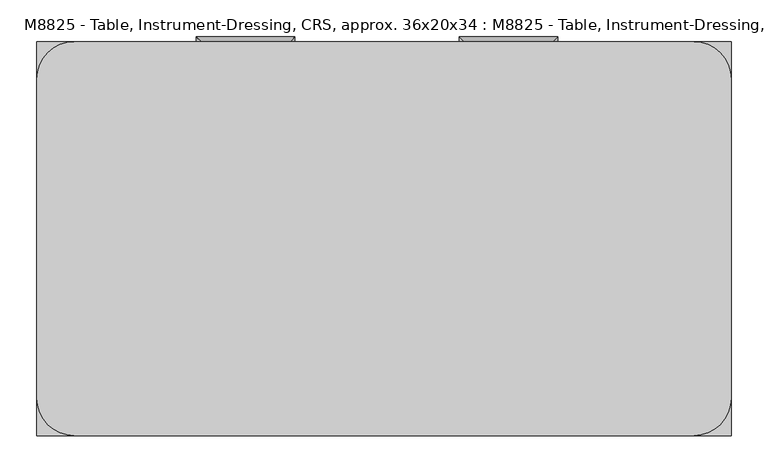
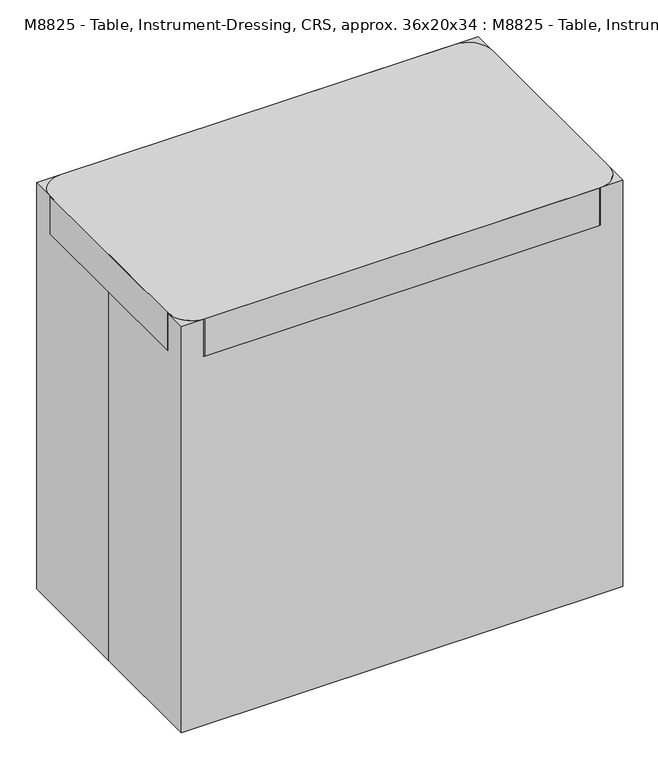
"""IFC4 building model written with IfcOpenShell, lengths in millimetres: proxy geometry, M8825 - Table, Instrument-Dressing, CRS, approx. 36x20x34 : M8825 - Table, Instrument-Dressing, CRS, approx. 36x20x34."""

import ifcopenshell
import ifcopenshell.guid

model = None  # the IFC model being written
_history = None  # IfcOwnerHistory: only IFC2X3 demands one
_inside = {}  # id of a spatial element -> (the spatial element, [elements in it])
_under = {}  # id of a project, library or spatial element -> (it, [spatial elements below it])
_declared = {}  # id of a project -> (the project, [libraries it declares])
_typed = {}  # id of a type object -> (the type object, [elements of that type])
_made_of = {}  # id of a material, layer set ... -> (it, [elements and type objects made of it])


def new_model(schema):
    """Start an empty IFC model of exactly this schema.

    Asked for "IFC4X3", IfcOpenShell would pick the latest addendum, in which some entities
    have other attributes; the version numbers below select the first issue.
    IFC2X3 requires an IfcOwnerHistory on every rooted entity: one is made here for all.
    """
    global model, _history
    if schema == "IFC4X3":
        model = ifcopenshell.file(schema_version=(4, 3, 0, 0))
    else:
        model = ifcopenshell.file(schema=schema)
    _inside.clear()
    _under.clear()
    _declared.clear()
    _typed.clear()
    _made_of.clear()
    _history = None
    if model.schema == "IFC2X3":
        org = make("IfcOrganization", Name="unknown")
        user = make(
            "IfcPersonAndOrganization",
            ThePerson=make("IfcPerson", FamilyName="unknown"),
            TheOrganization=org,
        )
        app = make(
            "IfcApplication",
            ApplicationDeveloper=org,
            Version="unknown",
            ApplicationFullName="unknown",
            ApplicationIdentifier="unknown",
        )
        _history = make(
            "IfcOwnerHistory",
            OwningUser=user,
            OwningApplication=app,
            ChangeAction="ADDED",
            CreationDate=0,
        )
    return model


def make(cls, **values):
    """One entity of the class cls with the attributes given. An attribute that is None is left unset."""
    return model.create_entity(
        cls, **{name: value for name, value in values.items() if value is not None}
    )


def rooted(cls, **values):
    """An entity with a GlobalId (a new one), such as an element, a storey or a relation."""
    return make(cls, GlobalId=ifcopenshell.guid.new(), OwnerHistory=_history, **values)


def si_unit(unit_type, name, prefix=None):
    """IfcSIUnit, for example si_unit("LENGTHUNIT", "METRE", prefix="MILLI")."""
    return make("IfcSIUnit", UnitType=unit_type, Prefix=prefix, Name=name)


def assignment(units):
    """IfcUnitAssignment: the units of a project."""
    return None if units is None else make("IfcUnitAssignment", Units=units)


def point(xyz):
    """IfcCartesianPoint."""
    return None if xyz is None else make("IfcCartesianPoint", Coordinates=xyz)


def direction(xyz):
    """IfcDirection."""
    return None if xyz is None else make("IfcDirection", DirectionRatios=xyz)


def frame(location, z_axis=None, x_axis=None):
    """IfcAxis2Placement3D, a coordinate frame: its origin and axes. An axis left out is left unset."""
    return make(
        "IfcAxis2Placement3D",
        Location=point(location),
        Axis=direction(z_axis),
        RefDirection=direction(x_axis),
    )


def frame_2d(location, x_axis=None):
    """IfcAxis2Placement2D, a coordinate frame in the plane: its origin and x axis."""
    return make(
        "IfcAxis2Placement2D", Location=point(location), RefDirection=direction(x_axis)
    )


def origin():
    """The frame at (0, 0, 0) with its axes left unset."""
    return frame((0.0, 0.0, 0.0))


def origin_with_axes():
    """The frame at (0, 0, 0) with the z axis (0, 0, 1) and the x axis (1, 0, 0) written out."""
    return frame((0.0, 0.0, 0.0), z_axis=(0.0, 0.0, 1.0), x_axis=(1.0, 0.0, 0.0))


def place(relative_to, where):
    """IfcLocalPlacement: puts the frame where relative to a parent placement (None: the world)."""
    return make(
        "IfcLocalPlacement", PlacementRelTo=relative_to, RelativePlacement=where
    )


def context(
    kind, dimensions, precision=None, world=None, true_north=None, identifier=None
):
    """IfcGeometricRepresentationContext, for example the 3D "Model" context."""
    return make(
        "IfcGeometricRepresentationContext",
        ContextIdentifier=identifier,
        ContextType=kind,
        CoordinateSpaceDimension=dimensions,
        Precision=precision,
        WorldCoordinateSystem=world,
        TrueNorth=true_north,
    )


def project(units=None, contexts=None):
    """IfcProject with its units and contexts."""
    return rooted(
        "IfcProject",
        Name="project",
        RepresentationContexts=contexts,
        UnitsInContext=assignment(units),
    )


def spatial(cls, under=None, at=None, **own):
    """A site, building, storey or space (cls), placed at a placement, below another one or the project."""
    s = rooted(cls, ObjectPlacement=at, **own)
    if under is not None:
        _under.setdefault(under.id(), (under, []))[1].append(s)
    return s


def polyline(points):
    """IfcPolyline through the points."""
    return make("IfcPolyline", Points=[point(p) for p in points])


def circle_curve(where, radius):
    """IfcCircle in the frame where."""
    return make("IfcCircle", Position=where, Radius=radius)


def ellipse_curve(where, semi_axis1, semi_axis2):
    """IfcEllipse in the frame where."""
    return make(
        "IfcEllipse", Position=where, SemiAxis1=semi_axis1, SemiAxis2=semi_axis2
    )


def trimmed(basis, trim1, trim2, sense, master):
    """IfcTrimmedCurve: the piece of a basis curve between two trims."""
    return make(
        "IfcTrimmedCurve",
        BasisCurve=basis,
        Trim1=trim1,
        Trim2=trim2,
        SenseAgreement=sense,
        MasterRepresentation=master,
    )


def segment(curve, same_sense, transition):
    """IfcCompositeCurveSegment."""
    return make(
        "IfcCompositeCurveSegment",
        Transition=transition,
        SameSense=same_sense,
        ParentCurve=curve,
    )


def composite_curve(segments, self_intersect=None):
    """IfcCompositeCurve: segments joined end to end."""
    return make("IfcCompositeCurve", Segments=segments, SelfIntersect=self_intersect)


def outline(outer, holes=None, kind="AREA"):
    """IfcArbitraryClosedProfileDef: a profile drawn as a closed curve; with holes, ...WithVoids."""
    if holes is None:
        return make("IfcArbitraryClosedProfileDef", ProfileType=kind, OuterCurve=outer)
    return make(
        "IfcArbitraryProfileDefWithVoids",
        ProfileType=kind,
        OuterCurve=outer,
        InnerCurves=holes,
    )


def extrude(swept, where, along, depth):
    """IfcExtrudedAreaSolid: the profile swept, set in the frame where, extruded along a direction by depth."""
    return make(
        "IfcExtrudedAreaSolid",
        SweptArea=swept,
        Position=where,
        ExtrudedDirection=direction(along),
        Depth=depth,
    )


def shape(context_of_items, identifier, shape_type, items):
    """IfcShapeRepresentation: the items that make up one representation, for example the "Body"."""
    return make(
        "IfcShapeRepresentation",
        ContextOfItems=context_of_items,
        RepresentationIdentifier=identifier,
        RepresentationType=shape_type,
        Items=items,
    )


def source(mapping_origin, context_of_items, identifier, shape_type, items):
    """IfcRepresentationMap: a shape defined once, which mapped items show again and again."""
    return make(
        "IfcRepresentationMap",
        MappingOrigin=mapping_origin,
        MappedRepresentation=shape(context_of_items, identifier, shape_type, items),
    )


def transform(
    local_origin,
    x_axis=None,
    y_axis=None,
    z_axis=None,
    scale=None,
    scale2=None,
    scale3=None,
    uniform=True,
):
    """IfcCartesianTransformationOperator3D, or its non-uniform kind. x_axis, y_axis, z_axis: its Axis1, 2, 3."""
    if uniform:
        return make(
            "IfcCartesianTransformationOperator3D",
            Axis1=direction(x_axis),
            Axis2=direction(y_axis),
            LocalOrigin=point(local_origin),
            Scale=scale,
            Axis3=direction(z_axis),
        )
    return make(
        "IfcCartesianTransformationOperator3DnonUniform",
        Axis1=direction(x_axis),
        Axis2=direction(y_axis),
        LocalOrigin=point(local_origin),
        Scale=scale,
        Axis3=direction(z_axis),
        Scale2=scale2,
        Scale3=scale3,
    )


def mapped(mapping_source, mapping_target):
    """IfcMappedItem: shows the shape of a source again, moved by a transform."""
    return make(
        "IfcMappedItem", MappingSource=mapping_source, MappingTarget=mapping_target
    )


def made_of(thing, what):
    """Note that an element or type object is made of a material, layer set ...; save() writes the relation."""
    if what is not None:
        _made_of.setdefault(what.id(), (what, []))[1].append(thing)
    return thing


def element(
    cls,
    number,
    at=None,
    inside=None,
    cuts=None,
    type_object=None,
    material=None,
    context=None,
    identifier="Body",
    shape_type=None,
    held_by="IfcProductDefinitionShape",
    body=None,
    shapes=None,
    **own,
):
    """One element of the class cls, such as IfcWall. Its Tag is "e" and its number.

    at: its placement. inside: the storey or other place that contains it. cuts: it is an
    opening in that element (IfcRelVoidsElement). A single representation is given by context,
    identifier, shape_type and body (its items); several are given by shapes. held_by: the class
    of the entity that holds the representations. save() writes the other relations.
    """
    e = rooted(cls, Tag="e%d" % number, ObjectPlacement=at, **own)
    if body is not None:
        shapes = [shape(context, identifier, shape_type, body)]
    if shapes is not None:
        e.Representation = make(held_by, Representations=shapes)
    if inside is not None:
        _inside.setdefault(inside.id(), (inside, []))[1].append(e)
    if cuts is not None:
        rooted(
            "IfcRelVoidsElement", RelatingBuildingElement=cuts, RelatedOpeningElement=e
        )
    if type_object is not None:
        _typed.setdefault(type_object.id(), (type_object, []))[1].append(e)
    return made_of(e, material)


def aggregate(whole, parts):
    """IfcRelAggregates: a whole, such as a stair, and the parts it consists of."""
    return rooted("IfcRelAggregates", RelatingObject=whole, RelatedObjects=parts)


def save(model, path):
    """Write the relations noted so far, then the file.

    IfcRelAggregates (storeys below a building ...), IfcRelContainedInSpatialStructure (elements
    in a storey), IfcRelDefinesByType, IfcRelAssociatesMaterial and IfcRelDeclares: one each for
    every whole, place, type object, material and project.
    """
    for whole, parts in _under.values():
        aggregate(whole, parts)
    for where, things in _inside.values():
        rooted(
            "IfcRelContainedInSpatialStructure",
            RelatedElements=things,
            RelatingStructure=where,
        )
    for kind, things in _typed.values():
        rooted("IfcRelDefinesByType", RelatedObjects=things, RelatingType=kind)
    for what, things in _made_of.values():
        rooted("IfcRelAssociatesMaterial", RelatedObjects=things, RelatingMaterial=what)
    for by, libraries in _declared.values():
        rooted("IfcRelDeclares", RelatingContext=by, RelatedDefinitions=libraries)
    model.write(path)


def plane_surface(at):
    """IfcPlane: the flat surface through the origin of the frame at, square to its z axis."""
    return make("IfcPlane", Position=at)


def cylinder_surface(at, radius):
    """IfcCylindricalSurface: all points at the distance radius from the z axis of the frame at."""
    return make("IfcCylindricalSurface", Position=at, Radius=radius)


def advanced_brep(points, edges, surfaces, faces):
    """IfcAdvancedBrep: a solid bounded by faces that lie on surfaces and meet in shared edges.

    An edge is (start, end): straight between two places in points (the first is 0);
    or (start, end, curve); or (start, end, curve, False) where it runs against its curve.
    A face is (place in surfaces, loops), or (place, loops, False) where it looks against
    its surface's normal. A loop lists edges by number (the first is 1), with a minus sign
    where the edge is run from its end to its start. The first loop is the outer one.
    """
    corners = [point(p) for p in points]
    vertices = [make("IfcVertexPoint", VertexGeometry=c) for c in corners]
    made = []
    for start, end, *more in edges:
        made.append(
            make(
                "IfcEdgeCurve",
                EdgeStart=vertices[start],
                EdgeEnd=vertices[end],
                EdgeGeometry=more[0] if more else make("IfcPolyline", Points=[corners[start], corners[end]]),
                SameSense=more[1] if len(more) > 1 else True,
            )
        )
    hull = []
    for where, loops, *sense in faces:
        bounds = []
        for j, loop in enumerate(loops):
            ring = [make("IfcOrientedEdge", EdgeElement=made[abs(k) - 1], Orientation=k > 0) for k in loop]
            bounds.append(
                make(
                    "IfcFaceOuterBound" if j == 0 else "IfcFaceBound",
                    Bound=make("IfcEdgeLoop", EdgeList=ring),
                    Orientation=True,
                )
            )
        hull.append(make("IfcAdvancedFace", Bounds=bounds, FaceSurface=surfaces[where], SameSense=sense[0] if sense else True))
    return make("IfcAdvancedBrep", Outer=make("IfcClosedShell", CfsFaces=hull))


def m8825_table_instrument_dressing_crs_approx_36x20x34_m8825_625bd398(model_context):
    return source(origin(), model_context, "Body", "SolidModel", [
        extrude(outline(polyline([(-349.25, -174.4117179), (-400.05, -174.4117179), (-400.05, 171.4283546), (-349.25, 171.4283546), (-349.25, 209.5283546), (349.25, 209.5283546), (349.25, 171.4283546), (400.05, 171.4283546), (400.05, -174.4117179), (349.25, -174.4117179), (349.25, -212.5117179), (-349.25, -212.5117179), (-349.25, -174.4117179)])), frame((0.0, 0.0, 292.1), z_axis=(0.0, 0.0, 1.0), x_axis=(1.0, 0.0, 0.0)), (0.0, 0.0, 1.0), 38.1),
        advanced_brep(
        [(101.6, 228.5783546, 755.65), (114.3, 228.5783546, 755.65), (114.3, 260.35, 755.65), (101.6, 273.05, 755.65), (222.25, 260.35, 755.65), (234.95, 273.05, 755.65), (234.95, 228.5783546, 755.65), (222.25, 228.5783546, 755.65)],
        [
            (0, 1, circle_curve(frame((107.95, 228.5783546, 755.65), z_axis=(0.0, -1.0, 0.0), x_axis=(1.0, 0.0, 0.0)), 6.35)),
            (1, 0, circle_curve(frame((107.95, 228.5783546, 755.65), z_axis=(0.0, -1.0, 0.0), x_axis=(1.0, 0.0, 0.0)), 6.35)),
            (1, 2),
            (2, 3, ellipse_curve(frame((107.95, 266.7, 755.65), z_axis=(-0.7071067811865457, -0.7071067811865492, 0.0), x_axis=(0.7071067811865491, -0.7071067811865458, 0.0)), 8.9802561, 6.35)),
            (3, 0),
            (3, 2, ellipse_curve(frame((107.95, 266.7, 755.65), z_axis=(-0.7071067811865457, -0.7071067811865492, 0.0), x_axis=(0.7071067811865491, -0.7071067811865458, 0.0)), 8.9802561, 6.35)),
            (2, 4),
            (4, 5, ellipse_curve(frame((228.6, 266.7, 755.65), z_axis=(-0.7071067811865492, 0.7071067811865457, 0.0), x_axis=(-0.7071067811865458, -0.7071067811865492, 0.0)), 8.9802561, 6.35)),
            (5, 3),
            (5, 4, ellipse_curve(frame((228.6, 266.7, 755.65), z_axis=(-0.7071067811865492, 0.7071067811865457, 0.0), x_axis=(-0.7071067811865458, -0.7071067811865492, 0.0)), 8.9802561, 6.35)),
            (6, 7, circle_curve(frame((228.6, 228.5783546, 755.65), z_axis=(0.0, -1.0, 0.0), x_axis=(-1.0, 0.0, 0.0)), 6.35)),
            (7, 6, circle_curve(frame((228.6, 228.5783546, 755.65), z_axis=(0.0, -1.0, 0.0), x_axis=(-1.0, 0.0, 0.0)), 6.35)),
            (4, 7),
            (6, 5),
        ],
        [
            plane_surface(frame((107.95, 228.5783546, 755.65), z_axis=(0.0, -1.0, 0.0), x_axis=(0.0, 0.0, 1.0))),
            cylinder_surface(frame((107.95, 228.5783546, 755.65), z_axis=(0.0, -1.0, 0.0), x_axis=(1.0, 0.0, 0.0)), 6.35),
            cylinder_surface(frame((107.95, 266.7, 755.65), z_axis=(-1.0, 0.0, 0.0), x_axis=(0.0, -1.0, 0.0)), 6.35),
            plane_surface(frame((228.6, 228.5783546, 755.65), z_axis=(0.0, -1.0, 0.0), x_axis=(0.0, 0.0, 1.0))),
            cylinder_surface(frame((228.6, 266.7, 755.65), z_axis=(0.0, 1.0, 0.0), x_axis=(-1.0, 0.0, 0.0)), 6.35),
        ],
        [
            (0, [[1, 2]]),
            (1, [[3, 4, 5, -2]]),
            (1, [[-5, 6, -3, -1]]),
            (2, [[7, 8, 9, -4]]),
            (2, [[-9, 10, -7, -6]]),
            (3, [[11, 12]]),
            (4, [[13, -11, 14, -8]]),
            (4, [[-14, -12, -13, -10]]),
        ],
    ),
        extrude(outline(polyline([(328.7951144, 228.5783546), (328.7951144, 209.5283546), (23.9951144, 209.5283546), (23.9951144, 228.5783546), (328.7951144, 228.5783546)])), frame((0.0, 0.0, 714.264534), z_axis=(0.0, 0.0, 1.0), x_axis=(1.0, 0.0, 0.0)), (0.0, 0.0, 1.0), 88.9),
        advanced_brep(
        [(-254.0, 228.5783546, 755.65), (-241.3, 228.5783546, 755.65), (-241.3, 260.35, 755.65), (-254.0, 273.05, 755.65), (-133.35, 260.35, 755.65), (-120.65, 273.05, 755.65), (-120.65, 228.5783546, 755.65), (-133.35, 228.5783546, 755.65)],
        [
            (0, 1, circle_curve(frame((-247.65, 228.5783546, 755.65), z_axis=(0.0, -1.0, 0.0), x_axis=(1.0, 0.0, 0.0)), 6.35)),
            (1, 0, circle_curve(frame((-247.65, 228.5783546, 755.65), z_axis=(0.0, -1.0, 0.0), x_axis=(1.0, 0.0, 0.0)), 6.35)),
            (1, 2),
            (2, 3, ellipse_curve(frame((-247.65, 266.7, 755.65), z_axis=(-0.7071067811865457, -0.7071067811865492, 0.0), x_axis=(0.7071067811865491, -0.7071067811865458, 0.0)), 8.9802561, 6.35)),
            (3, 0),
            (3, 2, ellipse_curve(frame((-247.65, 266.7, 755.65), z_axis=(-0.7071067811865457, -0.7071067811865492, 0.0), x_axis=(0.7071067811865491, -0.7071067811865458, 0.0)), 8.9802561, 6.35)),
            (2, 4),
            (4, 5, ellipse_curve(frame((-127.0, 266.7, 755.65), z_axis=(-0.7071067811865492, 0.7071067811865457, 0.0), x_axis=(-0.7071067811865458, -0.7071067811865492, 0.0)), 8.9802561, 6.35)),
            (5, 3),
            (5, 4, ellipse_curve(frame((-127.0, 266.7, 755.65), z_axis=(-0.7071067811865492, 0.7071067811865457, 0.0), x_axis=(-0.7071067811865458, -0.7071067811865492, 0.0)), 8.9802561, 6.35)),
            (6, 7, circle_curve(frame((-127.0, 228.5783546, 755.65), z_axis=(0.0, -1.0, 0.0), x_axis=(-1.0, 0.0, 0.0)), 6.35)),
            (7, 6, circle_curve(frame((-127.0, 228.5783546, 755.65), z_axis=(0.0, -1.0, 0.0), x_axis=(-1.0, 0.0, 0.0)), 6.35)),
            (4, 7),
            (6, 5),
        ],
        [
            plane_surface(frame((-247.65, 228.5783546, 755.65), z_axis=(0.0, -1.0, 0.0), x_axis=(0.0, 0.0, 1.0))),
            cylinder_surface(frame((-247.65, 228.5783546, 755.65), z_axis=(0.0, -1.0, 0.0), x_axis=(1.0, 0.0, 0.0)), 6.35),
            cylinder_surface(frame((-247.65, 266.7, 755.65), z_axis=(-1.0, 0.0, 0.0), x_axis=(0.0, -1.0, 0.0)), 6.35),
            plane_surface(frame((-127.0, 228.5783546, 755.65), z_axis=(0.0, -1.0, 0.0), x_axis=(0.0, 0.0, 1.0))),
            cylinder_surface(frame((-127.0, 266.7, 755.65), z_axis=(0.0, 1.0, 0.0), x_axis=(-1.0, 0.0, 0.0)), 6.35),
        ],
        [
            (0, [[1, 2]]),
            (1, [[3, 4, 5, -2]]),
            (1, [[-5, 6, -3, -1]]),
            (2, [[7, 8, 9, -4]]),
            (2, [[-9, 10, -7, -6]]),
            (3, [[11, 12]]),
            (4, [[13, -11, 14, -8]]),
            (4, [[-14, -12, -13, -10]]),
        ],
    ),
        extrude(outline(polyline([(-26.8048856, 228.5783546), (-26.8048856, 209.5283546), (-331.6048856, 209.5283546), (-331.6048856, 228.5783546), (-26.8048856, 228.5783546)])), frame((0.0, 0.0, 714.264534), z_axis=(0.0, 0.0, 1.0), x_axis=(1.0, 0.0, 0.0)), (0.0, 0.0, 1.0), 88.9),
        extrude(outline(polyline([(349.25, -193.4617179), (349.25, -212.5117179), (-349.25, -212.5117179), (-349.25, -193.4617179), (349.25, -193.4617179)])), frame((0.0, 0.0, 690.1016667), z_axis=(0.0, 0.0, 1.0), x_axis=(1.0, 0.0, 0.0)), (0.0, 0.0, 1.0), 139.7),
        extrude(outline(polyline([(349.25, 209.5283546), (349.25, 190.4783546), (-349.25, 190.4783546), (-349.25, 209.5283546), (349.25, 209.5283546)])), frame((0.0, 0.0, 690.1016667), z_axis=(0.0, 0.0, 1.0), x_axis=(1.0, 0.0, 0.0)), (0.0, 0.0, 1.0), 139.7),
        extrude(outline(polyline([(381.0, 171.4283546), (400.05, 171.4283546), (400.05, -174.4117179), (381.0, -174.4117179), (381.0, 171.4283546)])), frame((0.0, 0.0, 690.1016667), z_axis=(0.0, 0.0, 1.0), x_axis=(1.0, 0.0, 0.0)), (0.0, 0.0, 1.0), 139.7),
        extrude(outline(polyline([(-381.0, -174.4117179), (-400.05, -174.4117179), (-400.05, 171.4283546), (-381.0, 171.4283546), (-381.0, -174.4117179)])), frame((0.0, 0.0, 690.1016667), z_axis=(0.0, 0.0, 1.0), x_axis=(1.0, 0.0, 0.0)), (0.0, 0.0, 1.0), 139.7),
        extrude(outline(polyline([(349.25, 209.5283546), (400.05, 209.5283546), (400.05, 171.4283546), (349.25, 171.4283546), (349.25, 209.5283546)])), frame((0.0, 0.0, 127.0), z_axis=(0.0, 0.0, 1.0), x_axis=(1.0, 0.0, 0.0)), (0.0, 0.0, 1.0), 702.8016667),
        extrude(outline(polyline([(349.25, -212.5117179), (349.25, -174.4117179), (400.05, -174.4117179), (400.05, -212.5117179), (349.25, -212.5117179)])), frame((0.0, 0.0, 127.0), z_axis=(0.0, 0.0, 1.0), x_axis=(1.0, 0.0, 0.0)), (0.0, 0.0, 1.0), 702.8016667),
        extrude(outline(polyline([(-349.25, 209.5283546), (-349.25, 171.4283546), (-400.05, 171.4283546), (-400.05, 209.5283546), (-349.25, 209.5283546)])), frame((0.0, 0.0, 127.0), z_axis=(0.0, 0.0, 1.0), x_axis=(1.0, 0.0, 0.0)), (0.0, 0.0, 1.0), 702.8016667),
        extrude(outline(polyline([(-349.25, -212.5117179), (-400.05, -212.5117179), (-400.05, -174.4117179), (-349.25, -174.4117179), (-349.25, -212.5117179)])), frame((0.0, 0.0, 127.0), z_axis=(0.0, 0.0, 1.0), x_axis=(1.0, 0.0, 0.0)), (0.0, 0.0, 1.0), 702.8016667),
        extrude(outline(composite_curve([segment(trimmed(circle_curve(frame_2d((-366.1833333, -193.6533546)), 16.9333333), [point((-366.1833333, -210.5866879))], [point((-366.1833333, -176.7200213))], False, "CARTESIAN"), True, "CONTINUOUS"), segment(trimmed(circle_curve(frame_2d((-366.1833333, -193.6533546)), 16.9333333), [point((-366.1833333, -176.7200213))], [point((-366.1833333, -210.5866879))], False, "CARTESIAN"), True, "CONTINUOUS")], self_intersect=False)), frame((0.0, 0.0, 84.8149176), z_axis=(0.0, 0.0, 1.0), x_axis=(1.0, 0.0, 0.0)), (0.0, 0.0, 1.0), 42.1850824),
        extrude(outline(composite_curve([segment(trimmed(circle_curve(frame_2d((-366.1833333, 190.4783546)), 16.9333333), [point((-366.1833333, 207.4116879))], [point((-366.1833333, 173.5450213))], False, "CARTESIAN"), True, "CONTINUOUS"), segment(trimmed(circle_curve(frame_2d((-366.1833333, 190.4783546)), 16.9333333), [point((-366.1833333, 173.5450213))], [point((-366.1833333, 207.4116879))], False, "CARTESIAN"), True, "CONTINUOUS")], self_intersect=False)), frame((0.0, 0.0, 84.8149176), z_axis=(0.0, 0.0, 1.0), x_axis=(1.0, 0.0, 0.0)), (0.0, 0.0, 1.0), 42.1850824),
        extrude(outline(composite_curve([segment(trimmed(circle_curve(frame_2d((50.8, -349.25)), 50.8), [point((50.8, -400.05))], [point((50.8, -298.45))], False, "CARTESIAN"), True, "CONTINUOUS"), segment(trimmed(circle_curve(frame_2d((50.8, -349.25)), 50.8), [point((50.8, -298.45))], [point((50.8, -400.05))], False, "CARTESIAN"), True, "CONTINUOUS")], self_intersect=False)), frame((0.0, 152.4, 0.0), z_axis=(0.0, 1.0, 0.0), x_axis=(0.0, 0.0, 1.0)), (0.0, 0.0, 1.0), 19.05),
        extrude(outline(composite_curve([segment(trimmed(circle_curve(frame_2d((50.8, -349.25)), 50.8), [point((50.8, -400.05))], [point((50.8, -298.45))], False, "CARTESIAN"), True, "CONTINUOUS"), segment(trimmed(circle_curve(frame_2d((50.8, -349.25)), 50.8), [point((50.8, -298.45))], [point((50.8, -400.05))], False, "CARTESIAN"), True, "CONTINUOUS")], self_intersect=False)), frame((0.0, 209.55, 0.0), z_axis=(0.0, 1.0, 0.0), x_axis=(0.0, 0.0, 1.0)), (0.0, 0.0, 1.0), 19.05),
        extrude(outline(composite_curve([segment(trimmed(circle_curve(frame_2d((50.8, -349.25)), 33.8666667), [point((50.8, -315.3833333))], [point((50.8, -383.1166667))], False, "CARTESIAN"), True, "CONTINUOUS"), segment(trimmed(circle_curve(frame_2d((50.8, -349.25)), 33.8666667), [point((50.8, -383.1166667))], [point((50.8, -315.3833333))], False, "CARTESIAN"), True, "CONTINUOUS")], self_intersect=False)), frame((0.0, 171.45, 0.0), z_axis=(0.0, 1.0, 0.0), x_axis=(0.0, 0.0, 1.0)), (0.0, 0.0, 1.0), 38.1),
        extrude(outline(composite_curve([segment(trimmed(circle_curve(frame_2d((50.8, -349.25)), 50.8), [point((50.8, -400.05))], [point((50.8, -298.45))], False, "CARTESIAN"), True, "CONTINUOUS"), segment(trimmed(circle_curve(frame_2d((50.8, -349.25)), 50.8), [point((50.8, -298.45))], [point((50.8, -400.05))], False, "CARTESIAN"), True, "CONTINUOUS")], self_intersect=False)), frame((0.0, -174.4117179, 0.0), z_axis=(0.0, 1.0, 0.0), x_axis=(0.0, 0.0, 1.0)), (0.0, 0.0, 1.0), 19.05),
        extrude(outline(composite_curve([segment(trimmed(circle_curve(frame_2d((50.8, -349.25)), 50.8), [point((50.8, -400.05))], [point((50.8, -298.45))], False, "CARTESIAN"), True, "CONTINUOUS"), segment(trimmed(circle_curve(frame_2d((50.8, -349.25)), 50.8), [point((50.8, -298.45))], [point((50.8, -400.05))], False, "CARTESIAN"), True, "CONTINUOUS")], self_intersect=False)), frame((0.0, -231.5617179, 0.0), z_axis=(0.0, 1.0, 0.0), x_axis=(0.0, 0.0, 1.0)), (0.0, 0.0, 1.0), 19.05),
        extrude(outline(composite_curve([segment(trimmed(circle_curve(frame_2d((50.8, -349.25)), 33.8666667), [point((50.8, -315.3833333))], [point((50.8, -383.1166667))], False, "CARTESIAN"), True, "CONTINUOUS"), segment(trimmed(circle_curve(frame_2d((50.8, -349.25)), 33.8666667), [point((50.8, -383.1166667))], [point((50.8, -315.3833333))], False, "CARTESIAN"), True, "CONTINUOUS")], self_intersect=False)), frame((0.0, -212.5117179, 0.0), z_axis=(0.0, 1.0, 0.0), x_axis=(0.0, 0.0, 1.0)), (0.0, 0.0, 1.0), 38.1),
        extrude(outline(composite_curve([segment(trimmed(circle_curve(frame_2d((366.1833333, -193.6533546)), 16.9333333), [point((366.1833333, -210.5866879))], [point((366.1833333, -176.7200213))], False, "CARTESIAN"), True, "CONTINUOUS"), segment(trimmed(circle_curve(frame_2d((366.1833333, -193.6533546)), 16.9333333), [point((366.1833333, -176.7200213))], [point((366.1833333, -210.5866879))], False, "CARTESIAN"), True, "CONTINUOUS")], self_intersect=False)), frame((0.0, 0.0, 84.8149176), z_axis=(0.0, 0.0, 1.0), x_axis=(1.0, 0.0, 0.0)), (0.0, 0.0, 1.0), 42.1850824),
        extrude(outline(composite_curve([segment(trimmed(circle_curve(frame_2d((366.1833333, 190.4783546)), 16.9333333), [point((366.1833333, 207.4116879))], [point((366.1833333, 173.5450213))], False, "CARTESIAN"), True, "CONTINUOUS"), segment(trimmed(circle_curve(frame_2d((366.1833333, 190.4783546)), 16.9333333), [point((366.1833333, 173.5450213))], [point((366.1833333, 207.4116879))], False, "CARTESIAN"), True, "CONTINUOUS")], self_intersect=False)), frame((0.0, 0.0, 84.8149176), z_axis=(0.0, 0.0, 1.0), x_axis=(1.0, 0.0, 0.0)), (0.0, 0.0, 1.0), 42.1850824),
        extrude(outline(composite_curve([segment(trimmed(circle_curve(frame_2d((50.8, 349.25)), 50.8), [point((50.8, 400.05))], [point((50.8, 298.45))], False, "CARTESIAN"), True, "CONTINUOUS"), segment(trimmed(circle_curve(frame_2d((50.8, 349.25)), 50.8), [point((50.8, 298.45))], [point((50.8, 400.05))], False, "CARTESIAN"), True, "CONTINUOUS")], self_intersect=False)), frame((0.0, 152.4, 0.0), z_axis=(0.0, 1.0, 0.0), x_axis=(0.0, 0.0, 1.0)), (0.0, 0.0, 1.0), 19.05),
        extrude(outline(composite_curve([segment(trimmed(circle_curve(frame_2d((50.8, 349.25)), 50.8), [point((50.8, 400.05))], [point((50.8, 298.45))], False, "CARTESIAN"), True, "CONTINUOUS"), segment(trimmed(circle_curve(frame_2d((50.8, 349.25)), 50.8), [point((50.8, 298.45))], [point((50.8, 400.05))], False, "CARTESIAN"), True, "CONTINUOUS")], self_intersect=False)), frame((0.0, 209.55, 0.0), z_axis=(0.0, 1.0, 0.0), x_axis=(0.0, 0.0, 1.0)), (0.0, 0.0, 1.0), 19.05),
        extrude(outline(composite_curve([segment(trimmed(circle_curve(frame_2d((50.8, 349.25)), 33.8666667), [point((50.8, 315.3833333))], [point((50.8, 383.1166667))], False, "CARTESIAN"), True, "CONTINUOUS"), segment(trimmed(circle_curve(frame_2d((50.8, 349.25)), 33.8666667), [point((50.8, 383.1166667))], [point((50.8, 315.3833333))], False, "CARTESIAN"), True, "CONTINUOUS")], self_intersect=False)), frame((0.0, 171.45, 0.0), z_axis=(0.0, 1.0, 0.0), x_axis=(0.0, 0.0, 1.0)), (0.0, 0.0, 1.0), 38.1),
        extrude(outline(composite_curve([segment(trimmed(circle_curve(frame_2d((50.8, 349.25)), 50.8), [point((50.8, 400.05))], [point((50.8, 298.45))], False, "CARTESIAN"), True, "CONTINUOUS"), segment(trimmed(circle_curve(frame_2d((50.8, 349.25)), 50.8), [point((50.8, 298.45))], [point((50.8, 400.05))], False, "CARTESIAN"), True, "CONTINUOUS")], self_intersect=False)), frame((0.0, -174.4117179, 0.0), z_axis=(0.0, 1.0, 0.0), x_axis=(0.0, 0.0, 1.0)), (0.0, 0.0, 1.0), 19.05),
        extrude(outline(composite_curve([segment(trimmed(circle_curve(frame_2d((50.8, 349.25)), 50.8), [point((50.8, 400.05))], [point((50.8, 298.45))], False, "CARTESIAN"), True, "CONTINUOUS"), segment(trimmed(circle_curve(frame_2d((50.8, 349.25)), 50.8), [point((50.8, 298.45))], [point((50.8, 400.05))], False, "CARTESIAN"), True, "CONTINUOUS")], self_intersect=False)), frame((0.0, -231.5617179, 0.0), z_axis=(0.0, 1.0, 0.0), x_axis=(0.0, 0.0, 1.0)), (0.0, 0.0, 1.0), 19.05),
        extrude(outline(composite_curve([segment(trimmed(circle_curve(frame_2d((50.8, 349.25)), 33.8666667), [point((50.8, 315.3833333))], [point((50.8, 383.1166667))], False, "CARTESIAN"), True, "CONTINUOUS"), segment(trimmed(circle_curve(frame_2d((50.8, 349.25)), 33.8666667), [point((50.8, 383.1166667))], [point((50.8, 315.3833333))], False, "CARTESIAN"), True, "CONTINUOUS")], self_intersect=False)), frame((0.0, -212.5117179, 0.0), z_axis=(0.0, 1.0, 0.0), x_axis=(0.0, 0.0, 1.0)), (0.0, 0.0, 1.0), 38.1),
        extrude(outline(composite_curve([segment(polyline([(419.1, -266.7), (-419.1, -266.7)]), True, "CONTINUOUS"), segment(trimmed(circle_curve(frame_2d((-419.1, -215.9)), 50.8), [point((-419.1, -266.7))], [point((-469.9, -215.9))], False, "CARTESIAN"), True, "CONTINUOUS"), segment(polyline([(-469.9, -215.9), (-469.9, 215.9)]), True, "CONTINUOUS"), segment(trimmed(circle_curve(frame_2d((-419.1, 215.9)), 50.8), [point((-469.9, 215.9))], [point((-419.1, 266.7))], False, "CARTESIAN"), True, "CONTINUOUS"), segment(polyline([(-419.1, 266.7), (419.1, 266.7)]), True, "CONTINUOUS"), segment(trimmed(circle_curve(frame_2d((419.1, 215.9)), 50.8), [point((419.1, 266.7))], [point((469.9, 215.9))], False, "CARTESIAN"), True, "CONTINUOUS"), segment(polyline([(469.9, 215.9), (469.9, -215.9)]), True, "CONTINUOUS"), segment(trimmed(circle_curve(frame_2d((419.1, -215.9)), 50.8), [point((469.9, -215.9))], [point((419.1, -266.7))], False, "CARTESIAN"), True, "CONTINUOUS")], self_intersect=False)), frame((0.0, 0.0, 829.8016667), z_axis=(0.0, 0.0, 1.0), x_axis=(1.0, 0.0, 0.0)), (0.0, 0.0, 1.0), 84.5983333),
        extrude(outline(polyline([(-469.9, -266.7), (-469.9, 0.0), (-469.9, 266.7), (469.9, 266.7), (469.9, -266.7), (-469.9, -266.7)])), origin_with_axes(), (0.0, 0.0, 1.0), 914.4),
    ])


if __name__ == "__main__":
    model = new_model("IFC4")
    model_context = context("Model", 3, world=origin())
    ifc_project = project(units=[si_unit("LENGTHUNIT", "METRE", prefix="MILLI")], contexts=[model_context])
    site = spatial("IfcSite", under=ifc_project)
    building = spatial("IfcBuilding", under=site)
    placement = place(None, origin())
    m8825_table_instrument_dressing_crs_approx_36x20x34_m8825_shape = m8825_table_instrument_dressing_crs_approx_36x20x34_m8825_625bd398(model_context)
    element("IfcBuildingElementProxy", 1, Name="M8825 - Table, Instrument-Dressing, CRS, approx. 36x20x34 : M8825 - Table, Instrument-Dressing, CRS, approx. 36x20x34", ObjectType="M8825 - Table, Instrument-Dressing, CRS, approx. 36x20x34 : M8825 - Table, Instrument-Dressing, CRS, approx. 36x20x34", at=placement, inside=building, context=model_context, shape_type="MappedRepresentation", body=[
        mapped(m8825_table_instrument_dressing_crs_approx_36x20x34_m8825_shape, transform((0.0, 0.0, 0.0), x_axis=(1.0, 0.0, 0.0), y_axis=(0.0, 1.0, 0.0), z_axis=(0.0, 0.0, 1.0))),
    ])
    save(model, "model.ifc")

# Revit data of these elements
# Type "M8825 - Table, Instrument-Dressing, CRS, approx. 36x20x34 : M8825 - Table, Instrument-Dressing, CRS, approx. 36x20x34"
#   Watts2 = "0"
#   Watts1 = "0"
#   Unit_Issue = "EA"
#   UTIL_6_Misc = "-"
#   UTIL_5_NonMedGas = "-"
#   UTIL_4_MiscGas = "-"
#   UTIL_3_MedGas = "-"
#   UTIL_2_Elec = "-"
#   UTIL_1_WaterDrain = "-"
#   Nomenclature = "Table, Instrument/Dressing, CRS, approx. 36x20x34"
#   NSN = "6530"
#   Location [instance default] = ""
#   JSN = "M8825"
#   Fund_Source_VA = "-"
#   Fund_Source_Navy = "-"
#   Fund_Source_Army = "-"
#   Fund_Source_AF = "-"
#   ELEC_Volts2 = "0"
#   ELEC_Volts1 = "0"
#   ELEC_Phase2 = "0"
#   ELEC_Phase1 = "0"
#   ELEC_HertzSwitch = "0"
#   ELEC_HertzDependent = "0"
#   ELEC_Hertz = "0"
#   ELEC_Amps2 = "0"
#   ELEC_Amps1 = "0"
#   DetailDescription = "Instrument and dressing table. Made of corrosion resistant stainless steel with a sound deadened top. Includes guard rail, shelf and two side-by-side drawers. The table is mounted on swivel, ball-bearing casters."
#   CAT_VA = "C"
#   CAT_Navy = "C"
#   CAT_IHS = "-"
#   CAT_Army = "C"
#   CAT_AF = "C"
#   BTUperhour = "0"
#   radius = 0' - 2"
#   calc 2 = 0' - 0.66667"
#   calc 1 = 0' - 1.33333"
#   Weight_IP = 90
#   DIM_Width_IP = 3' - 1"
#   DIM_Height_IP = 3' - 0"
#   DIM_Depth_IP = 1' - 9"
#   top [instance default] = none
#   finish [instance default] = none
# Element 1 (IfcBuildingElementProxy, "M8825 - Table, Instrument-Dressing, CRS, approx. 36x20x34 : M8825 - Table, Instrument-Dressing, CRS, approx. 36x20x34")
#   Location = "ORCS1"
#   Materials on its faces: "EquipSpace"
# Materials
#   "EquipSpace": class "Unassigned", colour RGB 221 217 195, transparency 0.5
